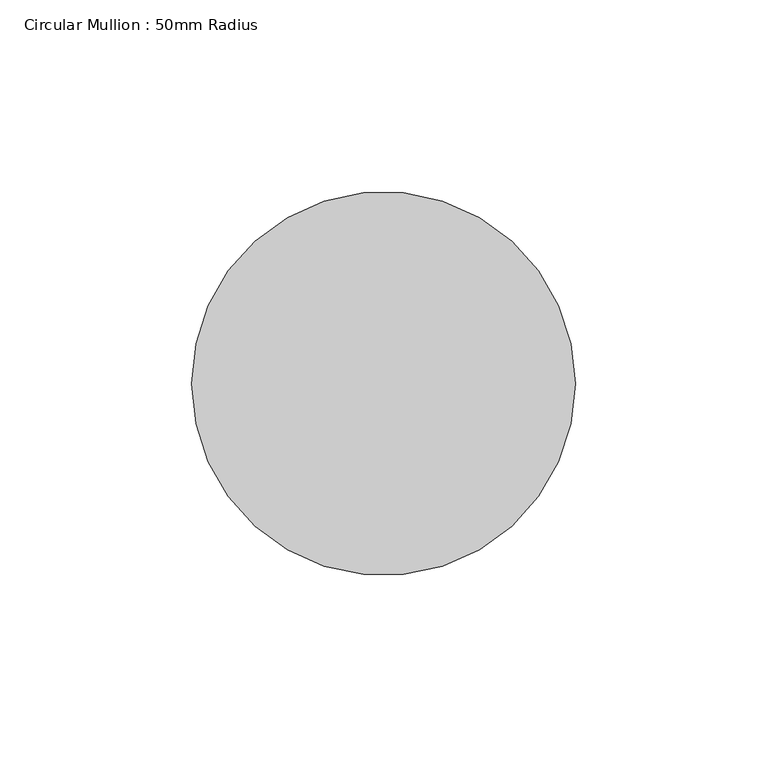
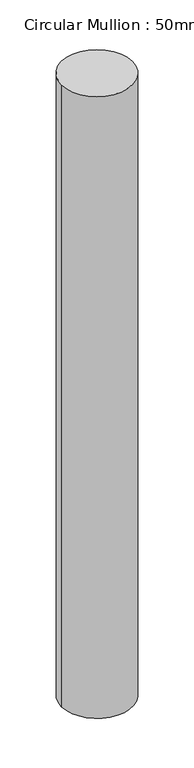
"""IFC4 building model written with IfcOpenShell, lengths in millimetres: member geometry, Circular Mullion : 50mm Radius."""

import ifcopenshell
import ifcopenshell.guid

model = None  # the IFC model being written
_history = None  # IfcOwnerHistory: only IFC2X3 demands one
_inside = {}  # id of a spatial element -> (the spatial element, [elements in it])
_under = {}  # id of a project, library or spatial element -> (it, [spatial elements below it])
_declared = {}  # id of a project -> (the project, [libraries it declares])
_typed = {}  # id of a type object -> (the type object, [elements of that type])
_made_of = {}  # id of a material, layer set ... -> (it, [elements and type objects made of it])


def new_model(schema):
    """Start an empty IFC model of exactly this schema.

    Asked for "IFC4X3", IfcOpenShell would pick the latest addendum, in which some entities
    have other attributes; the version numbers below select the first issue.
    IFC2X3 requires an IfcOwnerHistory on every rooted entity: one is made here for all.
    """
    global model, _history
    if schema == "IFC4X3":
        model = ifcopenshell.file(schema_version=(4, 3, 0, 0))
    else:
        model = ifcopenshell.file(schema=schema)
    _inside.clear()
    _under.clear()
    _declared.clear()
    _typed.clear()
    _made_of.clear()
    _history = None
    if model.schema == "IFC2X3":
        org = make("IfcOrganization", Name="unknown")
        user = make(
            "IfcPersonAndOrganization",
            ThePerson=make("IfcPerson", FamilyName="unknown"),
            TheOrganization=org,
        )
        app = make(
            "IfcApplication",
            ApplicationDeveloper=org,
            Version="unknown",
            ApplicationFullName="unknown",
            ApplicationIdentifier="unknown",
        )
        _history = make(
            "IfcOwnerHistory",
            OwningUser=user,
            OwningApplication=app,
            ChangeAction="ADDED",
            CreationDate=0,
        )
    return model


def make(cls, **values):
    """One entity of the class cls with the attributes given. An attribute that is None is left unset."""
    return model.create_entity(
        cls, **{name: value for name, value in values.items() if value is not None}
    )


def rooted(cls, **values):
    """An entity with a GlobalId (a new one), such as an element, a storey or a relation."""
    return make(cls, GlobalId=ifcopenshell.guid.new(), OwnerHistory=_history, **values)


def si_unit(unit_type, name, prefix=None):
    """IfcSIUnit, for example si_unit("LENGTHUNIT", "METRE", prefix="MILLI")."""
    return make("IfcSIUnit", UnitType=unit_type, Prefix=prefix, Name=name)


def assignment(units):
    """IfcUnitAssignment: the units of a project."""
    return None if units is None else make("IfcUnitAssignment", Units=units)


def point(xyz):
    """IfcCartesianPoint."""
    return None if xyz is None else make("IfcCartesianPoint", Coordinates=xyz)


def direction(xyz):
    """IfcDirection."""
    return None if xyz is None else make("IfcDirection", DirectionRatios=xyz)


def frame(location, z_axis=None, x_axis=None):
    """IfcAxis2Placement3D, a coordinate frame: its origin and axes. An axis left out is left unset."""
    return make(
        "IfcAxis2Placement3D",
        Location=point(location),
        Axis=direction(z_axis),
        RefDirection=direction(x_axis),
    )


def frame_2d(location, x_axis=None):
    """IfcAxis2Placement2D, a coordinate frame in the plane: its origin and x axis."""
    return make(
        "IfcAxis2Placement2D", Location=point(location), RefDirection=direction(x_axis)
    )


def origin():
    """The frame at (0, 0, 0) with its axes left unset."""
    return frame((0.0, 0.0, 0.0))


def origin_2d():
    """The frame at (0, 0) in the plane with its x axis left unset."""
    return frame_2d((0.0, 0.0))


def place(relative_to, where):
    """IfcLocalPlacement: puts the frame where relative to a parent placement (None: the world)."""
    return make(
        "IfcLocalPlacement", PlacementRelTo=relative_to, RelativePlacement=where
    )


def context(
    kind, dimensions, precision=None, world=None, true_north=None, identifier=None
):
    """IfcGeometricRepresentationContext, for example the 3D "Model" context."""
    return make(
        "IfcGeometricRepresentationContext",
        ContextIdentifier=identifier,
        ContextType=kind,
        CoordinateSpaceDimension=dimensions,
        Precision=precision,
        WorldCoordinateSystem=world,
        TrueNorth=true_north,
    )


def project(units=None, contexts=None):
    """IfcProject with its units and contexts."""
    return rooted(
        "IfcProject",
        Name="project",
        RepresentationContexts=contexts,
        UnitsInContext=assignment(units),
    )


def spatial(cls, under=None, at=None, **own):
    """A site, building, storey or space (cls), placed at a placement, below another one or the project."""
    s = rooted(cls, ObjectPlacement=at, **own)
    if under is not None:
        _under.setdefault(under.id(), (under, []))[1].append(s)
    return s


def circle_curve(where, radius):
    """IfcCircle in the frame where."""
    return make("IfcCircle", Position=where, Radius=radius)


def trimmed(basis, trim1, trim2, sense, master):
    """IfcTrimmedCurve: the piece of a basis curve between two trims."""
    return make(
        "IfcTrimmedCurve",
        BasisCurve=basis,
        Trim1=trim1,
        Trim2=trim2,
        SenseAgreement=sense,
        MasterRepresentation=master,
    )


def segment(curve, same_sense, transition):
    """IfcCompositeCurveSegment."""
    return make(
        "IfcCompositeCurveSegment",
        Transition=transition,
        SameSense=same_sense,
        ParentCurve=curve,
    )


def composite_curve(segments, self_intersect=None):
    """IfcCompositeCurve: segments joined end to end."""
    return make("IfcCompositeCurve", Segments=segments, SelfIntersect=self_intersect)


def outline(outer, holes=None, kind="AREA"):
    """IfcArbitraryClosedProfileDef: a profile drawn as a closed curve; with holes, ...WithVoids."""
    if holes is None:
        return make("IfcArbitraryClosedProfileDef", ProfileType=kind, OuterCurve=outer)
    return make(
        "IfcArbitraryProfileDefWithVoids",
        ProfileType=kind,
        OuterCurve=outer,
        InnerCurves=holes,
    )


def extrude(swept, where, along, depth):
    """IfcExtrudedAreaSolid: the profile swept, set in the frame where, extruded along a direction by depth."""
    return make(
        "IfcExtrudedAreaSolid",
        SweptArea=swept,
        Position=where,
        ExtrudedDirection=direction(along),
        Depth=depth,
    )


def shape(context_of_items, identifier, shape_type, items):
    """IfcShapeRepresentation: the items that make up one representation, for example the "Body"."""
    return make(
        "IfcShapeRepresentation",
        ContextOfItems=context_of_items,
        RepresentationIdentifier=identifier,
        RepresentationType=shape_type,
        Items=items,
    )


def source(mapping_origin, context_of_items, identifier, shape_type, items):
    """IfcRepresentationMap: a shape defined once, which mapped items show again and again."""
    return make(
        "IfcRepresentationMap",
        MappingOrigin=mapping_origin,
        MappedRepresentation=shape(context_of_items, identifier, shape_type, items),
    )


def transform(
    local_origin,
    x_axis=None,
    y_axis=None,
    z_axis=None,
    scale=None,
    scale2=None,
    scale3=None,
    uniform=True,
):
    """IfcCartesianTransformationOperator3D, or its non-uniform kind. x_axis, y_axis, z_axis: its Axis1, 2, 3."""
    if uniform:
        return make(
            "IfcCartesianTransformationOperator3D",
            Axis1=direction(x_axis),
            Axis2=direction(y_axis),
            LocalOrigin=point(local_origin),
            Scale=scale,
            Axis3=direction(z_axis),
        )
    return make(
        "IfcCartesianTransformationOperator3DnonUniform",
        Axis1=direction(x_axis),
        Axis2=direction(y_axis),
        LocalOrigin=point(local_origin),
        Scale=scale,
        Axis3=direction(z_axis),
        Scale2=scale2,
        Scale3=scale3,
    )


def mapped(mapping_source, mapping_target):
    """IfcMappedItem: shows the shape of a source again, moved by a transform."""
    return make(
        "IfcMappedItem", MappingSource=mapping_source, MappingTarget=mapping_target
    )


def made_of(thing, what):
    """Note that an element or type object is made of a material, layer set ...; save() writes the relation."""
    if what is not None:
        _made_of.setdefault(what.id(), (what, []))[1].append(thing)
    return thing


def element(
    cls,
    number,
    at=None,
    inside=None,
    cuts=None,
    type_object=None,
    material=None,
    context=None,
    identifier="Body",
    shape_type=None,
    held_by="IfcProductDefinitionShape",
    body=None,
    shapes=None,
    **own,
):
    """One element of the class cls, such as IfcWall. Its Tag is "e" and its number.

    at: its placement. inside: the storey or other place that contains it. cuts: it is an
    opening in that element (IfcRelVoidsElement). A single representation is given by context,
    identifier, shape_type and body (its items); several are given by shapes. held_by: the class
    of the entity that holds the representations. save() writes the other relations.
    """
    e = rooted(cls, Tag="e%d" % number, ObjectPlacement=at, **own)
    if body is not None:
        shapes = [shape(context, identifier, shape_type, body)]
    if shapes is not None:
        e.Representation = make(held_by, Representations=shapes)
    if inside is not None:
        _inside.setdefault(inside.id(), (inside, []))[1].append(e)
    if cuts is not None:
        rooted(
            "IfcRelVoidsElement", RelatingBuildingElement=cuts, RelatedOpeningElement=e
        )
    if type_object is not None:
        _typed.setdefault(type_object.id(), (type_object, []))[1].append(e)
    return made_of(e, material)


def aggregate(whole, parts):
    """IfcRelAggregates: a whole, such as a stair, and the parts it consists of."""
    return rooted("IfcRelAggregates", RelatingObject=whole, RelatedObjects=parts)


def save(model, path):
    """Write the relations noted so far, then the file.

    IfcRelAggregates (storeys below a building ...), IfcRelContainedInSpatialStructure (elements
    in a storey), IfcRelDefinesByType, IfcRelAssociatesMaterial and IfcRelDeclares: one each for
    every whole, place, type object, material and project.
    """
    for whole, parts in _under.values():
        aggregate(whole, parts)
    for where, things in _inside.values():
        rooted(
            "IfcRelContainedInSpatialStructure",
            RelatedElements=things,
            RelatingStructure=where,
        )
    for kind, things in _typed.values():
        rooted("IfcRelDefinesByType", RelatedObjects=things, RelatingType=kind)
    for what, things in _made_of.values():
        rooted("IfcRelAssociatesMaterial", RelatedObjects=things, RelatingMaterial=what)
    for by, libraries in _declared.values():
        rooted("IfcRelDeclares", RelatingContext=by, RelatedDefinitions=libraries)
    model.write(path)


def circular_mullion_50mm_radius_826fe490(model_context):
    return source(origin(), model_context, "Body", "SweptSolid", [
        extrude(outline(composite_curve([segment(trimmed(circle_curve(origin_2d(), 50.0), [point((50.0, 0.0))], [point((-50.0, 0.0))], False, "CARTESIAN"), True, "CONTINUOUS"), segment(trimmed(circle_curve(origin_2d(), 50.0), [point((-50.0, 0.0))], [point((50.0, 0.0))], False, "CARTESIAN"), True, "CONTINUOUS")], self_intersect=False)), frame((0.0, 0.0, -925.9926456), z_axis=(0.0, 0.0, 1.0), x_axis=(1.0, 0.0, 0.0)), (0.0, 0.0, 1.0), 925.9926456),
    ])


if __name__ == "__main__":
    model = new_model("IFC4")
    model_context = context("Model", 3, world=origin())
    ifc_project = project(units=[si_unit("LENGTHUNIT", "METRE", prefix="MILLI")], contexts=[model_context])
    site = spatial("IfcSite", under=ifc_project)
    building = spatial("IfcBuilding", under=site)
    placement = place(None, origin())
    circular_mullion_50mm_radius_shape = circular_mullion_50mm_radius_826fe490(model_context)
    element("IfcMember", 1, ObjectType="Circular Mullion : 50mm Radius", at=placement, inside=building, context=model_context, shape_type="MappedRepresentation", body=[
        mapped(circular_mullion_50mm_radius_shape, transform((0.0, 0.0, 0.0), x_axis=(1.0, 0.0, 0.0), y_axis=(0.0, 1.0, 0.0), z_axis=(0.0, 0.0, 1.0))),
    ])
    save(model, "model.ifc")

# Revit data of these elements
# Type "Circular Mullion : 50mm Radius"
#   built-in parameter 1007350 = 0.164042 (stored number, unit not read)
# Element 1 (IfcMember, "Circular Mullion : 50mm Radius")
#   Materials on its faces: "Aluminium"
# Materials
#   "Aluminium": class "Metal", colour RGB 247 247 247, transparency 0, Description = "Aluminium 6061", Cost = 0
